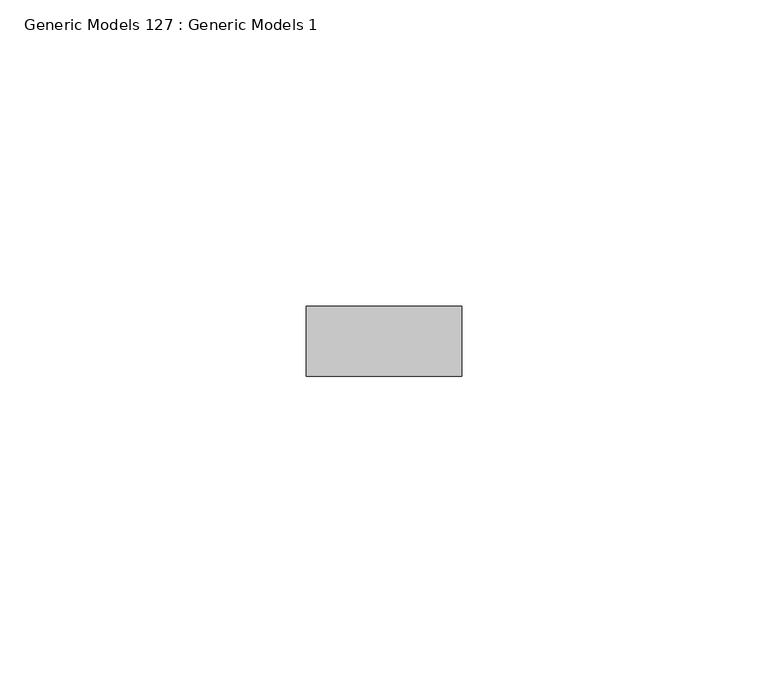
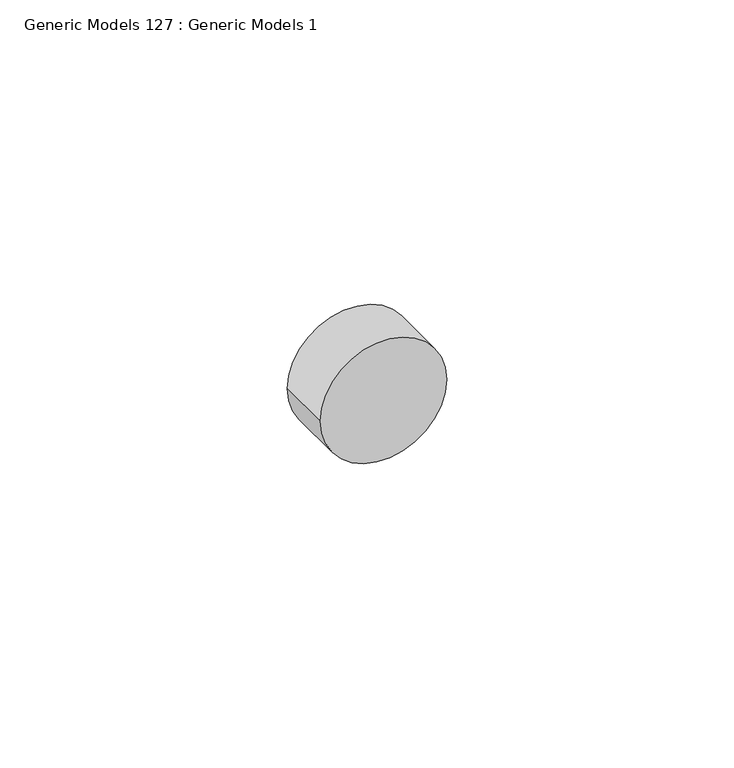
"""IFC4 building model written with IfcOpenShell, lengths in millimetres: proxy geometry, Generic Models 127 : Generic Models 1."""

from ifc_helpers import new_model, si_unit, point, frame, frame_2d, origin, place, context, project, spatial, circle_curve, trimmed, segment, composite_curve, outline, extrude, source, transform, mapped, element, save


def generic_models_127_generic_models_1_00b3787e(model_context):
    return source(origin(), model_context, "Body", "SweptSolid", [
        extrude(outline(composite_curve([segment(trimmed(circle_curve(frame_2d((38374.9548538, 7576.9346014)), 12.7), [point((38374.9548538, 7589.6346014))], [point((38374.9548538, 7564.2346014))], False, "CARTESIAN"), True, "CONTINUOUS"), segment(trimmed(circle_curve(frame_2d((38374.9548538, 7576.9346014)), 12.7), [point((38374.9548538, 7564.2346014))], [point((38374.9548538, 7589.6346014))], False, "CARTESIAN"), True, "CONTINUOUS")], self_intersect=False)), frame((0.0, 1836.9202358, 0.0), z_axis=(0.0, 1.0, 0.0), x_axis=(0.0, 0.0, 1.0)), (0.0, 0.0, 1.0), 11.4464372),
    ])


if __name__ == "__main__":
    model = new_model("IFC4")
    model_context = context("Model", 3, world=origin())
    ifc_project = project(units=[si_unit("LENGTHUNIT", "METRE", prefix="MILLI")], contexts=[model_context])
    site = spatial("IfcSite", under=ifc_project)
    building = spatial("IfcBuilding", under=site)
    placement = place(None, origin())
    generic_models_127_generic_models_1_shape = generic_models_127_generic_models_1_00b3787e(model_context)
    element("IfcBuildingElementProxy", 1, Name="Generic Models 127 : Generic Models 1", ObjectType="Generic Models 127 : Generic Models 1", at=placement, inside=building, context=model_context, shape_type="MappedRepresentation", body=[
        mapped(generic_models_127_generic_models_1_shape, transform((0.0, 0.0, 0.0), x_axis=(1.0, 0.0, 0.0), y_axis=(0.0, 1.0, 0.0), z_axis=(0.0, 0.0, 1.0))),
    ])
    save(model, "model.ifc")

# Revit data of these elements
# Project information
#   Issued Date 1 = "0/00/2018 - City of Newport Beach"
#   IfcSite GUID = "0g0KHFDXKHwQja200dNKHL"
#   IfcBuilding GUID = "0g0MjUDXKHwQM$200dNKHL"
#   IfcProject GUID = "3580753c_1e44_4e66_87a"
#   NameOverride = "Default Site"
#   Project Issue Date = "Issue Date"
#   Project Status = "Project Status"
#   Client Name = "xxx"
#   Project Address = "xxx"
#   Project Name = "STAUDENMEIER RESIDENCE"
# Element 1 (IfcBuildingElementProxy, "Generic Models 127 : Generic Models 1")
#   Materials on its faces: "S.S. LAG BOLT - SEE STRUCT. DWGS"
# Materials
#   "S.S. LAG BOLT - SEE STRUCT. DWGS": class "Generic", colour RGB 120 120 120, transparency 0, Cost = 0
